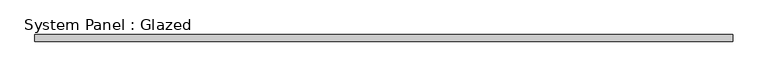
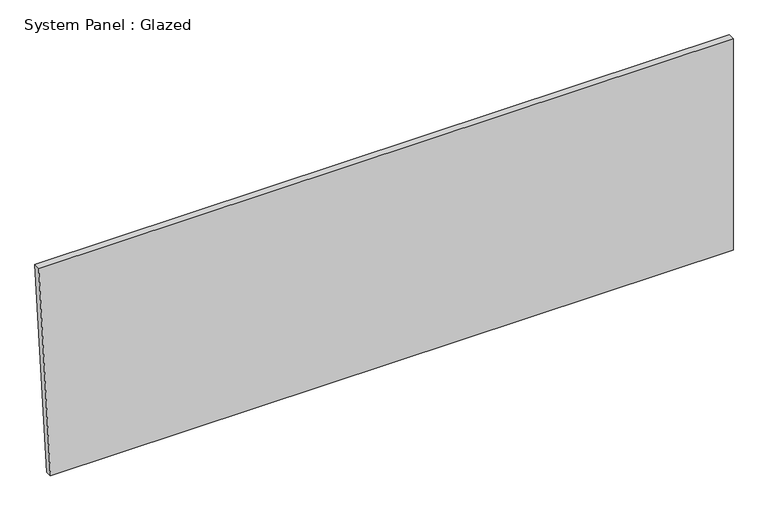
"""IFC4 building model written with IfcOpenShell, lengths in millimetres: plate geometry, System Panel : Glazed."""

from ifc_helpers import new_model, si_unit, frame, origin, place, context, project, spatial, polyline, outline, extrude, source, transform, mapped, element, save


def system_panel_glazed_cc02842b(model_context):
    return source(origin(), model_context, "Body", "SweptSolid", [
        extrude(outline(polyline([(0.0, -1297.8713084), (0.0, 1343.1943436), (866.0018549, 1343.1943436), (866.0018549, -1343.1943436), (0.0, -1297.8713084)])), frame((0.0, -44.45, 0.0), z_axis=(0.0, 1.0, 0.0), x_axis=(0.0, 0.0, 1.0)), (0.0, 0.0, 1.0), 25.4),
    ])


if __name__ == "__main__":
    model = new_model("IFC4")
    model_context = context("Model", 3, world=origin())
    ifc_project = project(units=[si_unit("LENGTHUNIT", "METRE", prefix="MILLI")], contexts=[model_context])
    site = spatial("IfcSite", under=ifc_project)
    building = spatial("IfcBuilding", under=site)
    placement = place(None, origin())
    system_panel_glazed_shape = system_panel_glazed_cc02842b(model_context)
    element("IfcPlate", 1, ObjectType="System Panel : Glazed", at=placement, inside=building, context=model_context, shape_type="MappedRepresentation", body=[
        mapped(system_panel_glazed_shape, transform((0.0, 0.0, 0.0), x_axis=(1.0, 0.0, 0.0), y_axis=(0.0, 1.0, 0.0), z_axis=(0.0, 0.0, 1.0))),
    ])
    save(model, "model.ifc")

# Revit data of these elements
# Type "System Panel : Glazed"
#   Construction Type Id = "GSP4R"
#   Analytic Construction = "1/8 in Pilkington single glazing"
#   Visual Light Transmittance = 0.9
#   Solar Heat Gain Coefficient = 0.86
#   Heat Transfer Coefficient (U) = 1.18115 BTU/(h·ft²·°F)
#   Define Thermal Properties by = 1
# Element 1 (IfcPlate, "System Panel : Glazed")
#   Materials on its faces: "Glass"
# Materials
#   "Glass": class "Glass", colour RGB 0 128 192, transparency 0.75, Description = "Soda Lime Glass", Cost = 0
